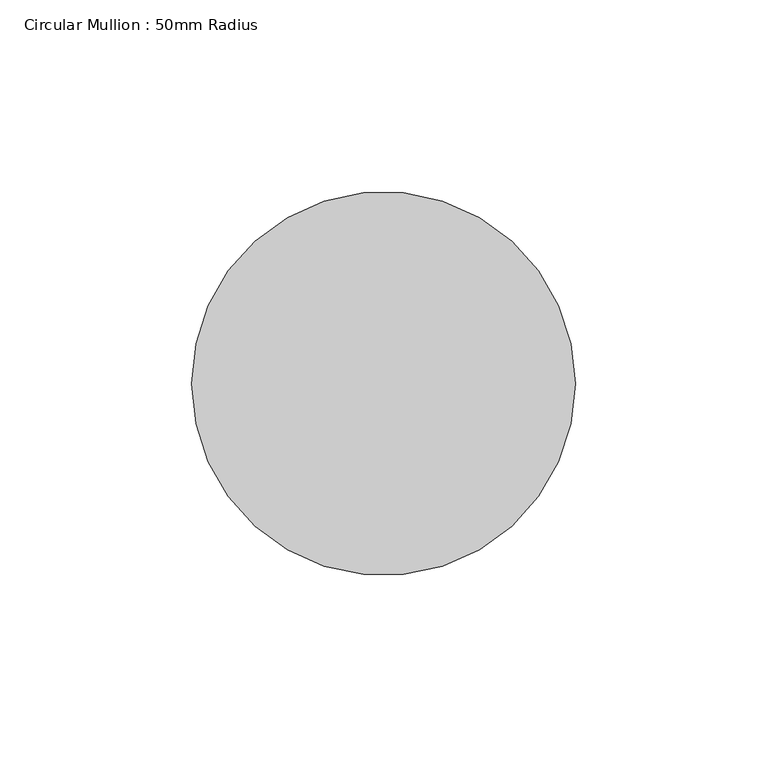
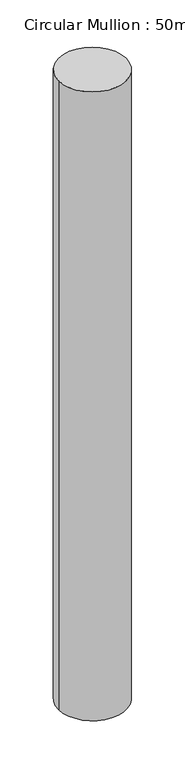
"""IFC4 building model written with IfcOpenShell, lengths in millimetres: member geometry, Circular Mullion : 50mm Radius."""

import ifcopenshell
import ifcopenshell.guid

model = None  # the IFC model being written
_history = None  # IfcOwnerHistory: only IFC2X3 demands one
_inside = {}  # id of a spatial element -> (the spatial element, [elements in it])
_under = {}  # id of a project, library or spatial element -> (it, [spatial elements below it])
_declared = {}  # id of a project -> (the project, [libraries it declares])
_typed = {}  # id of a type object -> (the type object, [elements of that type])
_made_of = {}  # id of a material, layer set ... -> (it, [elements and type objects made of it])


def new_model(schema):
    """Start an empty IFC model of exactly this schema.

    Asked for "IFC4X3", IfcOpenShell would pick the latest addendum, in which some entities
    have other attributes; the version numbers below select the first issue.
    IFC2X3 requires an IfcOwnerHistory on every rooted entity: one is made here for all.
    """
    global model, _history
    if schema == "IFC4X3":
        model = ifcopenshell.file(schema_version=(4, 3, 0, 0))
    else:
        model = ifcopenshell.file(schema=schema)
    _inside.clear()
    _under.clear()
    _declared.clear()
    _typed.clear()
    _made_of.clear()
    _history = None
    if model.schema == "IFC2X3":
        org = make("IfcOrganization", Name="unknown")
        user = make(
            "IfcPersonAndOrganization",
            ThePerson=make("IfcPerson", FamilyName="unknown"),
            TheOrganization=org,
        )
        app = make(
            "IfcApplication",
            ApplicationDeveloper=org,
            Version="unknown",
            ApplicationFullName="unknown",
            ApplicationIdentifier="unknown",
        )
        _history = make(
            "IfcOwnerHistory",
            OwningUser=user,
            OwningApplication=app,
            ChangeAction="ADDED",
            CreationDate=0,
        )
    return model


def make(cls, **values):
    """One entity of the class cls with the attributes given. An attribute that is None is left unset."""
    return model.create_entity(
        cls, **{name: value for name, value in values.items() if value is not None}
    )


def rooted(cls, **values):
    """An entity with a GlobalId (a new one), such as an element, a storey or a relation."""
    return make(cls, GlobalId=ifcopenshell.guid.new(), OwnerHistory=_history, **values)


def si_unit(unit_type, name, prefix=None):
    """IfcSIUnit, for example si_unit("LENGTHUNIT", "METRE", prefix="MILLI")."""
    return make("IfcSIUnit", UnitType=unit_type, Prefix=prefix, Name=name)


def assignment(units):
    """IfcUnitAssignment: the units of a project."""
    return None if units is None else make("IfcUnitAssignment", Units=units)


def point(xyz):
    """IfcCartesianPoint."""
    return None if xyz is None else make("IfcCartesianPoint", Coordinates=xyz)


def direction(xyz):
    """IfcDirection."""
    return None if xyz is None else make("IfcDirection", DirectionRatios=xyz)


def frame(location, z_axis=None, x_axis=None):
    """IfcAxis2Placement3D, a coordinate frame: its origin and axes. An axis left out is left unset."""
    return make(
        "IfcAxis2Placement3D",
        Location=point(location),
        Axis=direction(z_axis),
        RefDirection=direction(x_axis),
    )


def frame_2d(location, x_axis=None):
    """IfcAxis2Placement2D, a coordinate frame in the plane: its origin and x axis."""
    return make(
        "IfcAxis2Placement2D", Location=point(location), RefDirection=direction(x_axis)
    )


def origin():
    """The frame at (0, 0, 0) with its axes left unset."""
    return frame((0.0, 0.0, 0.0))


def origin_2d():
    """The frame at (0, 0) in the plane with its x axis left unset."""
    return frame_2d((0.0, 0.0))


def place(relative_to, where):
    """IfcLocalPlacement: puts the frame where relative to a parent placement (None: the world)."""
    return make(
        "IfcLocalPlacement", PlacementRelTo=relative_to, RelativePlacement=where
    )


def context(
    kind, dimensions, precision=None, world=None, true_north=None, identifier=None
):
    """IfcGeometricRepresentationContext, for example the 3D "Model" context."""
    return make(
        "IfcGeometricRepresentationContext",
        ContextIdentifier=identifier,
        ContextType=kind,
        CoordinateSpaceDimension=dimensions,
        Precision=precision,
        WorldCoordinateSystem=world,
        TrueNorth=true_north,
    )


def project(units=None, contexts=None):
    """IfcProject with its units and contexts."""
    return rooted(
        "IfcProject",
        Name="project",
        RepresentationContexts=contexts,
        UnitsInContext=assignment(units),
    )


def spatial(cls, under=None, at=None, **own):
    """A site, building, storey or space (cls), placed at a placement, below another one or the project."""
    s = rooted(cls, ObjectPlacement=at, **own)
    if under is not None:
        _under.setdefault(under.id(), (under, []))[1].append(s)
    return s


def circle_curve(where, radius):
    """IfcCircle in the frame where."""
    return make("IfcCircle", Position=where, Radius=radius)


def trimmed(basis, trim1, trim2, sense, master):
    """IfcTrimmedCurve: the piece of a basis curve between two trims."""
    return make(
        "IfcTrimmedCurve",
        BasisCurve=basis,
        Trim1=trim1,
        Trim2=trim2,
        SenseAgreement=sense,
        MasterRepresentation=master,
    )


def segment(curve, same_sense, transition):
    """IfcCompositeCurveSegment."""
    return make(
        "IfcCompositeCurveSegment",
        Transition=transition,
        SameSense=same_sense,
        ParentCurve=curve,
    )


def composite_curve(segments, self_intersect=None):
    """IfcCompositeCurve: segments joined end to end."""
    return make("IfcCompositeCurve", Segments=segments, SelfIntersect=self_intersect)


def outline(outer, holes=None, kind="AREA"):
    """IfcArbitraryClosedProfileDef: a profile drawn as a closed curve; with holes, ...WithVoids."""
    if holes is None:
        return make("IfcArbitraryClosedProfileDef", ProfileType=kind, OuterCurve=outer)
    return make(
        "IfcArbitraryProfileDefWithVoids",
        ProfileType=kind,
        OuterCurve=outer,
        InnerCurves=holes,
    )


def extrude(swept, where, along, depth):
    """IfcExtrudedAreaSolid: the profile swept, set in the frame where, extruded along a direction by depth."""
    return make(
        "IfcExtrudedAreaSolid",
        SweptArea=swept,
        Position=where,
        ExtrudedDirection=direction(along),
        Depth=depth,
    )


def shape(context_of_items, identifier, shape_type, items):
    """IfcShapeRepresentation: the items that make up one representation, for example the "Body"."""
    return make(
        "IfcShapeRepresentation",
        ContextOfItems=context_of_items,
        RepresentationIdentifier=identifier,
        RepresentationType=shape_type,
        Items=items,
    )


def source(mapping_origin, context_of_items, identifier, shape_type, items):
    """IfcRepresentationMap: a shape defined once, which mapped items show again and again."""
    return make(
        "IfcRepresentationMap",
        MappingOrigin=mapping_origin,
        MappedRepresentation=shape(context_of_items, identifier, shape_type, items),
    )


def transform(
    local_origin,
    x_axis=None,
    y_axis=None,
    z_axis=None,
    scale=None,
    scale2=None,
    scale3=None,
    uniform=True,
):
    """IfcCartesianTransformationOperator3D, or its non-uniform kind. x_axis, y_axis, z_axis: its Axis1, 2, 3."""
    if uniform:
        return make(
            "IfcCartesianTransformationOperator3D",
            Axis1=direction(x_axis),
            Axis2=direction(y_axis),
            LocalOrigin=point(local_origin),
            Scale=scale,
            Axis3=direction(z_axis),
        )
    return make(
        "IfcCartesianTransformationOperator3DnonUniform",
        Axis1=direction(x_axis),
        Axis2=direction(y_axis),
        LocalOrigin=point(local_origin),
        Scale=scale,
        Axis3=direction(z_axis),
        Scale2=scale2,
        Scale3=scale3,
    )


def mapped(mapping_source, mapping_target):
    """IfcMappedItem: shows the shape of a source again, moved by a transform."""
    return make(
        "IfcMappedItem", MappingSource=mapping_source, MappingTarget=mapping_target
    )


def made_of(thing, what):
    """Note that an element or type object is made of a material, layer set ...; save() writes the relation."""
    if what is not None:
        _made_of.setdefault(what.id(), (what, []))[1].append(thing)
    return thing


def element(
    cls,
    number,
    at=None,
    inside=None,
    cuts=None,
    type_object=None,
    material=None,
    context=None,
    identifier="Body",
    shape_type=None,
    held_by="IfcProductDefinitionShape",
    body=None,
    shapes=None,
    **own,
):
    """One element of the class cls, such as IfcWall. Its Tag is "e" and its number.

    at: its placement. inside: the storey or other place that contains it. cuts: it is an
    opening in that element (IfcRelVoidsElement). A single representation is given by context,
    identifier, shape_type and body (its items); several are given by shapes. held_by: the class
    of the entity that holds the representations. save() writes the other relations.
    """
    e = rooted(cls, Tag="e%d" % number, ObjectPlacement=at, **own)
    if body is not None:
        shapes = [shape(context, identifier, shape_type, body)]
    if shapes is not None:
        e.Representation = make(held_by, Representations=shapes)
    if inside is not None:
        _inside.setdefault(inside.id(), (inside, []))[1].append(e)
    if cuts is not None:
        rooted(
            "IfcRelVoidsElement", RelatingBuildingElement=cuts, RelatedOpeningElement=e
        )
    if type_object is not None:
        _typed.setdefault(type_object.id(), (type_object, []))[1].append(e)
    return made_of(e, material)


def aggregate(whole, parts):
    """IfcRelAggregates: a whole, such as a stair, and the parts it consists of."""
    return rooted("IfcRelAggregates", RelatingObject=whole, RelatedObjects=parts)


def save(model, path):
    """Write the relations noted so far, then the file.

    IfcRelAggregates (storeys below a building ...), IfcRelContainedInSpatialStructure (elements
    in a storey), IfcRelDefinesByType, IfcRelAssociatesMaterial and IfcRelDeclares: one each for
    every whole, place, type object, material and project.
    """
    for whole, parts in _under.values():
        aggregate(whole, parts)
    for where, things in _inside.values():
        rooted(
            "IfcRelContainedInSpatialStructure",
            RelatedElements=things,
            RelatingStructure=where,
        )
    for kind, things in _typed.values():
        rooted("IfcRelDefinesByType", RelatedObjects=things, RelatingType=kind)
    for what, things in _made_of.values():
        rooted("IfcRelAssociatesMaterial", RelatedObjects=things, RelatingMaterial=what)
    for by, libraries in _declared.values():
        rooted("IfcRelDeclares", RelatingContext=by, RelatedDefinitions=libraries)
    model.write(path)


def circular_mullion_50mm_radius_07cc004d(model_context):
    return source(origin(), model_context, "Body", "SweptSolid", [
        extrude(outline(composite_curve([segment(trimmed(circle_curve(origin_2d(), 50.0), [point((50.0, 0.0))], [point((-50.0, 0.0))], False, "CARTESIAN"), True, "CONTINUOUS"), segment(trimmed(circle_curve(origin_2d(), 50.0), [point((-50.0, 0.0))], [point((50.0, 0.0))], False, "CARTESIAN"), True, "CONTINUOUS")], self_intersect=False)), frame((0.0, 0.0, -983.7587033), z_axis=(0.0, 0.0, 1.0), x_axis=(1.0, 0.0, 0.0)), (0.0, 0.0, 1.0), 983.7587033),
    ])


if __name__ == "__main__":
    model = new_model("IFC4")
    model_context = context("Model", 3, world=origin())
    ifc_project = project(units=[si_unit("LENGTHUNIT", "METRE", prefix="MILLI")], contexts=[model_context])
    site = spatial("IfcSite", under=ifc_project)
    building = spatial("IfcBuilding", under=site)
    placement = place(None, origin())
    circular_mullion_50mm_radius_shape = circular_mullion_50mm_radius_07cc004d(model_context)
    element("IfcMember", 1, ObjectType="Circular Mullion : 50mm Radius", at=placement, inside=building, context=model_context, shape_type="MappedRepresentation", body=[
        mapped(circular_mullion_50mm_radius_shape, transform((0.0, 0.0, 0.0), x_axis=(1.0, 0.0, 0.0), y_axis=(0.0, 1.0, 0.0), z_axis=(0.0, 0.0, 1.0))),
    ])
    save(model, "model.ifc")

# Revit data of these elements
# Type "Circular Mullion : 50mm Radius"
#   built-in parameter 1007350 = 0.164042 (stored number, unit not read)
# Element 1 (IfcMember, "Circular Mullion : 50mm Radius")
#   Materials on its faces: "Aluminium"
# Materials
#   "Aluminium": class "Metal", colour RGB 247 247 247, transparency 0, Description = "Aluminium 6061", Cost = 0
